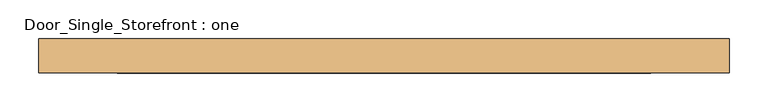
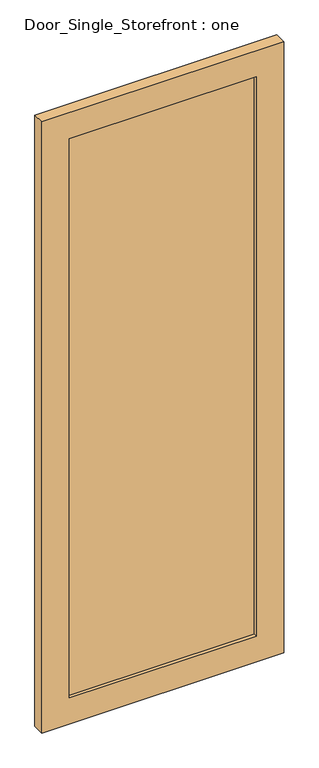
"""IFC4 building model written with IfcOpenShell, lengths in millimetres: door geometry, Door_Single_Storefront : one."""

from ifc_helpers import new_model, si_unit, frame, origin, place, context, project, spatial, polyline, outline, extrude, source, transform, mapped, element, save


def door_single_storefront_one_50b7ac91(model_context):
    return source(origin(), model_context, "Body", "SweptSolid", [
        extrude(outline(polyline([(2387.6, -446.88125), (0.0, -446.88125), (0.0, 446.88125), (2387.6, 446.88125), (2387.6, -446.88125)]), holes=[polyline([(101.6, 345.28125), (101.6, -345.28125), (2286.0, -345.28125), (2286.0, 345.28125), (101.6, 345.28125)])]), frame((0.0, -25.4, 0.0), z_axis=(0.0, 1.0, 0.0), x_axis=(0.0, 0.0, 1.0)), (0.0, 0.0, 1.0), 44.45),
        extrude(outline(polyline([(345.28125, 6.35), (345.28125, -12.7), (-345.28125, -12.7), (-345.28125, 6.35), (345.28125, 6.35)])), frame((0.0, 0.0, 101.6), z_axis=(0.0, 0.0, 1.0), x_axis=(1.0, 0.0, 0.0)), (0.0, 0.0, 1.0), 2184.4),
    ])


if __name__ == "__main__":
    model = new_model("IFC4")
    model_context = context("Model", 3, world=origin())
    ifc_project = project(units=[si_unit("LENGTHUNIT", "METRE", prefix="MILLI")], contexts=[model_context])
    site = spatial("IfcSite", under=ifc_project)
    building = spatial("IfcBuilding", under=site)
    placement = place(None, origin())
    door_single_storefront_one_shape = door_single_storefront_one_50b7ac91(model_context)
    element("IfcDoor", 1, ObjectType="Door_Single_Storefront : one", at=placement, inside=building, context=model_context, shape_type="MappedRepresentation", body=[
        mapped(door_single_storefront_one_shape, transform((0.0, 0.0, 0.0), x_axis=(1.0, 0.0, 0.0), y_axis=(0.0, 1.0, 0.0), z_axis=(0.0, 0.0, 1.0))),
    ])
    save(model, "model.ifc")

# Revit data of these elements
# Type "Door_Single_Storefront : one"
#   Type Mark = "27"
#   Analytic Construction = "<None>"
#   Stile_Width = 0' - 4"
#   Door_Thickness = 0' - 1 3/4"
#   Door_Offset = 0' - 1"
#   Glass_Material = Glass
#   Frame_Material = Aluminum
#   Function = (empty or 0)
# Element 1 (IfcDoor, "Door_Single_Storefront : one")
#   Materials on its faces: "Aluminum", "Glass"
# Materials
#   "Glass": class "Glass", colour RGB 142 168 196, transparency 0.75, Description = "Soda Lime Glass", Cost = 0
#   "Aluminum": class "Metal", colour RGB 226 226 226, transparency 0, Description = "Aluminum 6061", Cost = 0
